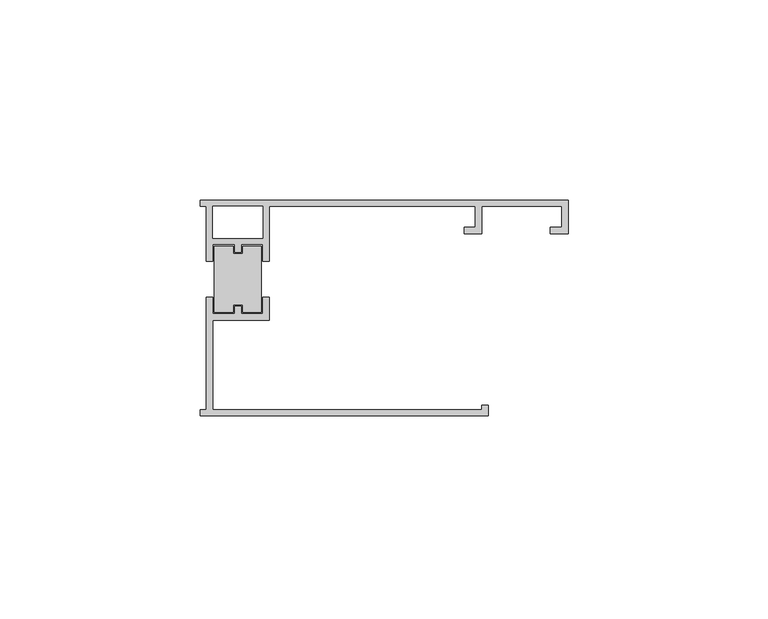
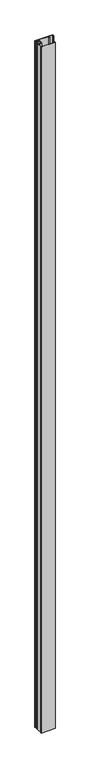
"""IFC4 building model written with IfcOpenShell, lengths in millimetres: proxy geometry, Generic Models 2:Generic Models 2:310765:Generic Models 2:310765 : Generic Models 2:Generic Models 2:310765:55 : Generic Models 2:Generic Models 2:310765:Generic Models 2:310765 : Generic Models 2:Generic Models 2:310765:300385."""

from ifc_helpers import new_model, si_unit, frame, origin, place, context, project, spatial, polyline, outline, extrude, source, transform, mapped, element, save


def generic_models_bdd2eba5(model_context):
    return source(origin(), model_context, "Body", "SweptSolid", [
        extrude(outline(polyline([(593397.4901937, -568246.416762), (593392.7926951, -568246.416762), (593392.7926951, -568244.4913465), (593390.4114451, -568244.4913465), (593390.4114451, -568246.416762), (593385.7139465, -568246.416762), (593385.7139465, -568229.8645058), (593390.4114451, -568229.8645058), (593390.4114451, -568231.7899212), (593392.7926951, -568231.7899212), (593392.7926951, -568229.8645058), (593397.4901937, -568229.8645058), (593397.4901937, -568246.416762)])), frame((0.0, 0.0, 4860.0679991), z_axis=(0.0, 0.0, 1.0), x_axis=(1.0, 0.0, 0.0)), (0.0, 0.0, 1.0), 3695.7),
        extrude(outline(polyline([(593474.1420715, -568226.7958673), (593469.7547449, -568226.7958673), (593469.7547449, -568225.2083673), (593472.5545715, -568225.2083673), (593472.5545715, -568219.9369958), (593452.5545715, -568219.9369958), (593452.5545715, -568226.7958673), (593448.1672449, -568226.7958673), (593448.1672449, -568225.2083673), (593450.9670715, -568225.2083673), (593450.9670715, -568219.9369958), (593399.4745688, -568219.9369958), (593399.4745688, -568233.6348183), (593397.8870688, -568233.6348183), (593397.8870688, -568229.4676308), (593392.3958201, -568229.4676308), (593392.3958201, -568231.3930462), (593390.8083201, -568231.3930462), (593390.8083201, -568229.4676308), (593385.3170715, -568229.4676308), (593385.3170715, -568233.6348183), (593383.7295715, -568233.6348183), (593383.7295715, -568219.9369958), (593382.1420715, -568219.9369958), (593382.1420715, -568218.3494958), (593474.1420715, -568218.3494958), (593474.1420715, -568226.7958673)]), holes=[polyline([(593397.8870688, -568219.9369958), (593385.3170715, -568219.9369958), (593385.3170715, -568227.8801308), (593397.8870688, -568227.8801308), (593397.8870688, -568219.9369958)])]), frame((0.0, 0.0, 4860.0679991), z_axis=(0.0, 0.0, 1.0), x_axis=(1.0, 0.0, 0.0)), (0.0, 0.0, 1.0), 3695.7),
        extrude(outline(polyline([(593382.1420715, -568270.7619958), (593383.7295715, -568270.7619958), (593383.7295715, -568242.6464495), (593385.3170715, -568242.6464495), (593385.3170715, -568246.813637), (593390.8083201, -568246.813637), (593390.8083201, -568244.8882215), (593392.3958201, -568244.8882215), (593392.3958201, -568246.813637), (593397.8870688, -568246.813637), (593397.8870688, -568242.6464495), (593399.4745688, -568242.6464495), (593399.4745688, -568248.401137), (593385.3170715, -568248.401137), (593385.3170715, -568270.7619958), (593452.5545715, -568270.7619958), (593452.5545715, -568269.6344059), (593454.1420715, -568269.6344059), (593454.1420715, -568272.3494958), (593382.1420715, -568272.3494958), (593382.1420715, -568270.7619958)])), frame((0.0, 0.0, 4860.0679991), z_axis=(0.0, 0.0, 1.0), x_axis=(1.0, 0.0, 0.0)), (0.0, 0.0, 1.0), 3695.7),
    ])


if __name__ == "__main__":
    model = new_model("IFC4")
    model_context = context("Model", 3, world=origin())
    ifc_project = project(units=[si_unit("LENGTHUNIT", "METRE", prefix="MILLI")], contexts=[model_context])
    site = spatial("IfcSite", under=ifc_project)
    building = spatial("IfcBuilding", under=site)
    placement = place(None, origin())
    generic_models_shape = generic_models_bdd2eba5(model_context)
    element("IfcBuildingElementProxy", 1, Name="Generic Models 2:Generic Models 2:310765:Generic Models 2:310765 : Generic Models 2:Generic Models 2:310765:55 : Generic Models 2:Generic Models 2:310765:Generic Models 2:310765 : Generic Models 2:Generic Models 2:310765:300385", ObjectType="Generic Models 2:Generic Models 2:310765:Generic Models 2:310765 : Generic Models 2:Generic Models 2:310765:55 : Generic Models 2:Generic Models 2:310765:Generic Models 2:310765 : Generic Models 2:Generic Models 2:310765:300385", at=placement, inside=building, context=model_context, shape_type="MappedRepresentation", body=[
        mapped(generic_models_shape, transform((0.0, 0.0, 0.0), x_axis=(1.0, 0.0, 0.0), y_axis=(0.0, 1.0, 0.0), z_axis=(0.0, 0.0, 1.0))),
    ])
    save(model, "model.ifc")

# Revit data of these elements
# Type "Generic Models 2:Generic Models 2:310765:Generic Models 2:310765 : Generic Models 2:Generic Models 2:310765:55 : Generic Models 2:Generic Models 2:310765:Generic Models 2:310765 : Generic Models 2:Generic Models 2:310765:300385"
#   NameOverride = "Generic Models 2:Generic Models 2:310765:Generic Models 2:310765 : Generic Models 2:Generic Models 2:310765:300385"
#   ObjectTypeOverride = "Generic Models 2:310765 : Generic Models 2:Generic Models 2:310765"
#   Reference = "Generic Models 2"
#   Tag = "300385"
# Element 1 (IfcBuildingElementProxy, "Generic Models 2:Generic Models 2:310765:Generic Models 2:310765 : Generic Models 2:Generic Models 2:310765:55 : Generic Models 2:Generic Models 2:310765:Generic Models 2:310765 : Generic Models 2:Generic Models 2:310765:300385")
#   Materials on its faces: "THERMAL BROKEN ALUMINUM STOREFRONT FOR POLYCARBONATE"
# Materials
#   "THERMAL BROKEN ALUMINUM STOREFRONT FOR POLYCARBONATE": class "Unassigned", colour RGB 244 244 244, transparency 0, Keynote = "M07611300.01", Cost = 0
